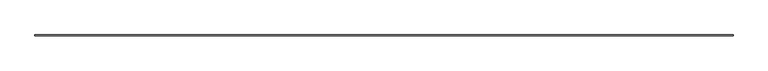
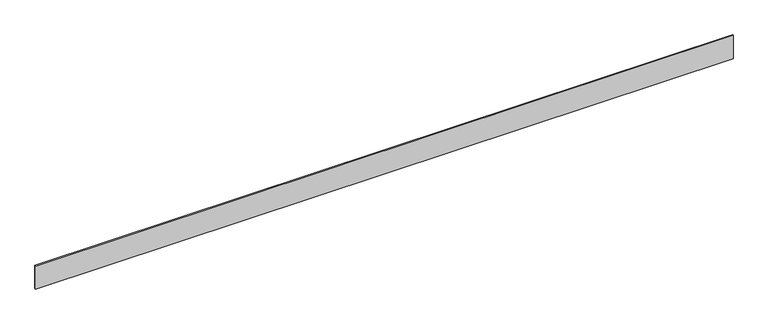
"""IFC4 building model written with IfcOpenShell, lengths in millimetres: proxy geometry, Generic Models 7:Generic Models 1:6:Generic Models 1:6 : Generic Models 7:Generic Models 1:337419:6 : Generic Models 7:Generic Models 1:6:Generic Models 1:6 : Generic Models 7:Generic Models 1:337419:312901."""

from ifc_helpers import new_model, si_unit, frame, origin, place, context, project, spatial, polyline, outline, extrude, source, transform, mapped, element, save


def generic_models_852af830(model_context):
    return source(origin(), model_context, "Body", "SweptSolid", [
        extrude(outline(polyline([(-536557.2913358, -3.1687897), (-536506.4913358, -5.2854564), (-536506.4913358, -1222.375), (-536557.2913358, -1222.375), (-536557.2913358, -3.1687897)])), frame((557809.7867239, 0.0, 0.0), z_axis=(1.0, 0.0, 0.0), x_axis=(0.0, 1.0, 0.0)), (0.0, 0.0, 1.0), 34892.5709653),
    ])


if __name__ == "__main__":
    model = new_model("IFC4")
    model_context = context("Model", 3, world=origin())
    ifc_project = project(units=[si_unit("LENGTHUNIT", "METRE", prefix="MILLI")], contexts=[model_context])
    site = spatial("IfcSite", under=ifc_project)
    building = spatial("IfcBuilding", under=site)
    placement = place(None, origin())
    generic_models_shape = generic_models_852af830(model_context)
    element("IfcBuildingElementProxy", 1, Name="Generic Models 7:Generic Models 1:6:Generic Models 1:6 : Generic Models 7:Generic Models 1:337419:6 : Generic Models 7:Generic Models 1:6:Generic Models 1:6 : Generic Models 7:Generic Models 1:337419:312901", ObjectType="Generic Models 7:Generic Models 1:6:Generic Models 1:6 : Generic Models 7:Generic Models 1:337419:6 : Generic Models 7:Generic Models 1:6:Generic Models 1:6 : Generic Models 7:Generic Models 1:337419:312901", at=placement, inside=building, context=model_context, shape_type="MappedRepresentation", body=[
        mapped(generic_models_shape, transform((0.0, 0.0, 0.0), x_axis=(1.0, 0.0, 0.0), y_axis=(0.0, 1.0, 0.0), z_axis=(0.0, 0.0, 1.0))),
    ])
    save(model, "model.ifc")

# Revit data of these elements
# Type "Generic Models 7:Generic Models 1:6:Generic Models 1:6 : Generic Models 7:Generic Models 1:337419:6 : Generic Models 7:Generic Models 1:6:Generic Models 1:6 : Generic Models 7:Generic Models 1:337419:312901"
#   NameOverride = "Generic Models 7:Generic Models 1:6:Generic Models 1:6 : Generic Models 7:Generic Models 1:337419:312901"
#   ObjectTypeOverride = "Generic Models 1:6 : Generic Models 7:Generic Models 1:337419"
#   Reference = "Generic Models 1"
#   Tag = "312901"
# Element 1 (IfcBuildingElementProxy, "Generic Models 7:Generic Models 1:6:Generic Models 1:6 : Generic Models 7:Generic Models 1:337419:6 : Generic Models 7:Generic Models 1:6:Generic Models 1:6 : Generic Models 7:Generic Models 1:337419:312901")
#   Materials on its faces: "EXTRUDED POLYSTYRENE (XPS) RIGID FOAM INSULATION (FOAMULAR® 250 OR SIMILAR)"
# Materials
#   "EXTRUDED POLYSTYRENE (XPS) RIGID FOAM INSULATION (FOAMULAR® 250 OR SIMILAR)": class "Unassigned", colour RGB 247 185 194, transparency 0, Cost = 0
